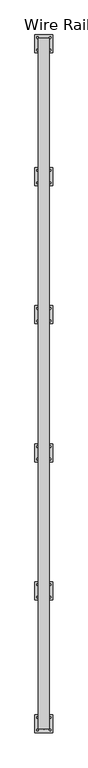
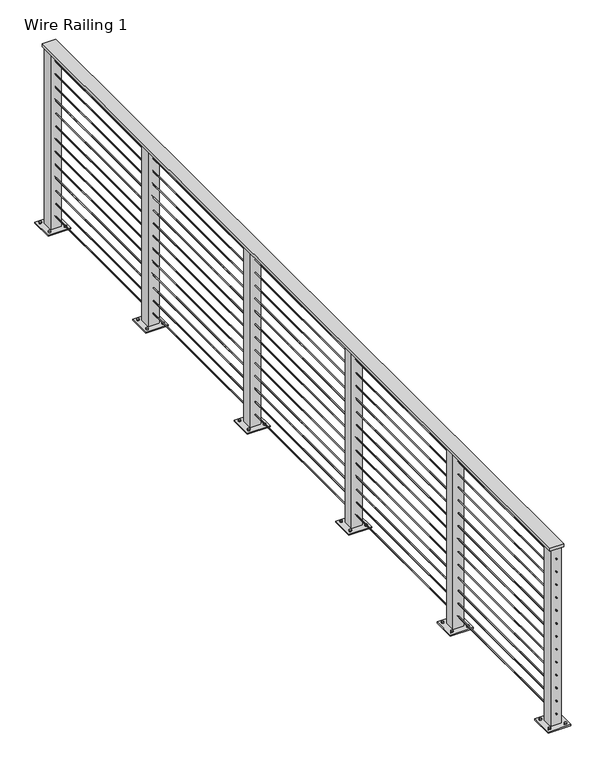
"""IFC4 building model written with IfcOpenShell, lengths in millimetres: railing geometry, Wire Railing 1."""

from ifc_helpers import new_model, si_unit, point, frame, frame_2d, origin, place, context, project, spatial, polyline, circle_curve, trimmed, segment, composite_curve, outline, extrude, source, transform, mapped, element, save


def wire_railing_1_036b5bdb(model_context):
    return source(origin(), model_context, "Body", "SweptSolid", [
        extrude(outline(polyline([(33186.6840778, 35113.0784511), (33262.8840778, 35113.0784511), (33262.8840778, 30205.3668167), (33186.6840778, 30205.3668167), (33186.6840778, 35113.0784511)])), frame((0.0, 0.0, 267442.95), z_axis=(0.0, 0.0, 1.0), x_axis=(1.0, 0.0, 0.0)), (0.0, 0.0, 1.0), 19.05),
        extrude(outline(composite_curve([segment(trimmed(circle_curve(frame_2d((267383.41875, 33224.7840778)), 2.38125), [point((267383.41875, 33227.1653278))], [point((267383.41875, 33222.4028278))], False, "CARTESIAN"), True, "CONTINUOUS"), segment(trimmed(circle_curve(frame_2d((267383.41875, 33224.7840778)), 2.38125), [point((267383.41875, 33222.4028278))], [point((267383.41875, 33227.1653278))], False, "CARTESIAN"), True, "CONTINUOUS")], self_intersect=False)), frame((0.0, 30205.3668167, 0.0), z_axis=(0.0, 1.0, 0.0), x_axis=(0.0, 0.0, 1.0)), (0.0, 0.0, 1.0), 4907.7116344),
        extrude(outline(composite_curve([segment(trimmed(circle_curve(frame_2d((267307.21875, 33224.7840778)), 2.38125), [point((267307.21875, 33227.1653278))], [point((267307.21875, 33222.4028278))], False, "CARTESIAN"), True, "CONTINUOUS"), segment(trimmed(circle_curve(frame_2d((267307.21875, 33224.7840778)), 2.38125), [point((267307.21875, 33222.4028278))], [point((267307.21875, 33227.1653278))], False, "CARTESIAN"), True, "CONTINUOUS")], self_intersect=False)), frame((0.0, 30205.3668167, 0.0), z_axis=(0.0, 1.0, 0.0), x_axis=(0.0, 0.0, 1.0)), (0.0, 0.0, 1.0), 4907.7116344),
        extrude(outline(composite_curve([segment(trimmed(circle_curve(frame_2d((267231.01875, 33224.7840778)), 2.38125), [point((267231.01875, 33227.1653278))], [point((267231.01875, 33222.4028278))], False, "CARTESIAN"), True, "CONTINUOUS"), segment(trimmed(circle_curve(frame_2d((267231.01875, 33224.7840778)), 2.38125), [point((267231.01875, 33222.4028278))], [point((267231.01875, 33227.1653278))], False, "CARTESIAN"), True, "CONTINUOUS")], self_intersect=False)), frame((0.0, 30205.3668167, 0.0), z_axis=(0.0, 1.0, 0.0), x_axis=(0.0, 0.0, 1.0)), (0.0, 0.0, 1.0), 4907.7116344),
        extrude(outline(composite_curve([segment(trimmed(circle_curve(frame_2d((267154.81875, 33224.7840778)), 2.38125), [point((267154.81875, 33227.1653278))], [point((267154.81875, 33222.4028278))], False, "CARTESIAN"), True, "CONTINUOUS"), segment(trimmed(circle_curve(frame_2d((267154.81875, 33224.7840778)), 2.38125), [point((267154.81875, 33222.4028278))], [point((267154.81875, 33227.1653278))], False, "CARTESIAN"), True, "CONTINUOUS")], self_intersect=False)), frame((0.0, 30205.3668167, 0.0), z_axis=(0.0, 1.0, 0.0), x_axis=(0.0, 0.0, 1.0)), (0.0, 0.0, 1.0), 4907.7116344),
        extrude(outline(composite_curve([segment(trimmed(circle_curve(frame_2d((267078.61875, 33224.7840778)), 2.38125), [point((267078.61875, 33227.1653278))], [point((267078.61875, 33222.4028278))], False, "CARTESIAN"), True, "CONTINUOUS"), segment(trimmed(circle_curve(frame_2d((267078.61875, 33224.7840778)), 2.38125), [point((267078.61875, 33222.4028278))], [point((267078.61875, 33227.1653278))], False, "CARTESIAN"), True, "CONTINUOUS")], self_intersect=False)), frame((0.0, 30205.3668167, 0.0), z_axis=(0.0, 1.0, 0.0), x_axis=(0.0, 0.0, 1.0)), (0.0, 0.0, 1.0), 4907.7116344),
        extrude(outline(composite_curve([segment(trimmed(circle_curve(frame_2d((267002.41875, 33224.7840778)), 2.38125), [point((267002.41875, 33227.1653278))], [point((267002.41875, 33222.4028278))], False, "CARTESIAN"), True, "CONTINUOUS"), segment(trimmed(circle_curve(frame_2d((267002.41875, 33224.7840778)), 2.38125), [point((267002.41875, 33222.4028278))], [point((267002.41875, 33227.1653278))], False, "CARTESIAN"), True, "CONTINUOUS")], self_intersect=False)), frame((0.0, 30205.3668167, 0.0), z_axis=(0.0, 1.0, 0.0), x_axis=(0.0, 0.0, 1.0)), (0.0, 0.0, 1.0), 4907.7116344),
        extrude(outline(composite_curve([segment(trimmed(circle_curve(frame_2d((266926.21875, 33224.7840778)), 2.38125), [point((266926.21875, 33227.1653278))], [point((266926.21875, 33222.4028278))], False, "CARTESIAN"), True, "CONTINUOUS"), segment(trimmed(circle_curve(frame_2d((266926.21875, 33224.7840778)), 2.38125), [point((266926.21875, 33222.4028278))], [point((266926.21875, 33227.1653278))], False, "CARTESIAN"), True, "CONTINUOUS")], self_intersect=False)), frame((0.0, 30205.3668167, 0.0), z_axis=(0.0, 1.0, 0.0), x_axis=(0.0, 0.0, 1.0)), (0.0, 0.0, 1.0), 4907.7116344),
        extrude(outline(composite_curve([segment(trimmed(circle_curve(frame_2d((266850.01875, 33224.7840778)), 2.38125), [point((266850.01875, 33227.1653278))], [point((266850.01875, 33222.4028278))], False, "CARTESIAN"), True, "CONTINUOUS"), segment(trimmed(circle_curve(frame_2d((266850.01875, 33224.7840778)), 2.38125), [point((266850.01875, 33222.4028278))], [point((266850.01875, 33227.1653278))], False, "CARTESIAN"), True, "CONTINUOUS")], self_intersect=False)), frame((0.0, 30205.3668167, 0.0), z_axis=(0.0, 1.0, 0.0), x_axis=(0.0, 0.0, 1.0)), (0.0, 0.0, 1.0), 4907.7116344),
        extrude(outline(composite_curve([segment(trimmed(circle_curve(frame_2d((266773.81875, 33224.7840778)), 2.38125), [point((266773.81875, 33227.1653278))], [point((266773.81875, 33222.4028278))], False, "CARTESIAN"), True, "CONTINUOUS"), segment(trimmed(circle_curve(frame_2d((266773.81875, 33224.7840778)), 2.38125), [point((266773.81875, 33222.4028278))], [point((266773.81875, 33227.1653278))], False, "CARTESIAN"), True, "CONTINUOUS")], self_intersect=False)), frame((0.0, 30205.3668167, 0.0), z_axis=(0.0, 1.0, 0.0), x_axis=(0.0, 0.0, 1.0)), (0.0, 0.0, 1.0), 4907.7116344),
        extrude(outline(composite_curve([segment(trimmed(circle_curve(frame_2d((266697.61875, 33224.7840778)), 2.38125), [point((266697.61875, 33227.1653278))], [point((266697.61875, 33222.4028278))], False, "CARTESIAN"), True, "CONTINUOUS"), segment(trimmed(circle_curve(frame_2d((266697.61875, 33224.7840778)), 2.38125), [point((266697.61875, 33222.4028278))], [point((266697.61875, 33227.1653278))], False, "CARTESIAN"), True, "CONTINUOUS")], self_intersect=False)), frame((0.0, 30205.3668167, 0.0), z_axis=(0.0, 1.0, 0.0), x_axis=(0.0, 0.0, 1.0)), (0.0, 0.0, 1.0), 4907.7116344),
        extrude(outline(composite_curve([segment(trimmed(circle_curve(frame_2d((266621.41875, 33224.7840778)), 2.38125), [point((266621.41875, 33227.1653278))], [point((266621.41875, 33222.4028278))], False, "CARTESIAN"), True, "CONTINUOUS"), segment(trimmed(circle_curve(frame_2d((266621.41875, 33224.7840778)), 2.38125), [point((266621.41875, 33222.4028278))], [point((266621.41875, 33227.1653278))], False, "CARTESIAN"), True, "CONTINUOUS")], self_intersect=False)), frame((0.0, 30205.3668167, 0.0), z_axis=(0.0, 1.0, 0.0), x_axis=(0.0, 0.0, 1.0)), (0.0, 0.0, 1.0), 4907.7116344),
        extrude(outline(composite_curve([segment(trimmed(circle_curve(frame_2d((266545.21875, 33224.7840778)), 2.38125), [point((266545.21875, 33227.1653278))], [point((266545.21875, 33222.4028278))], False, "CARTESIAN"), True, "CONTINUOUS"), segment(trimmed(circle_curve(frame_2d((266545.21875, 33224.7840778)), 2.38125), [point((266545.21875, 33222.4028278))], [point((266545.21875, 33227.1653278))], False, "CARTESIAN"), True, "CONTINUOUS")], self_intersect=False)), frame((0.0, 30205.3668167, 0.0), z_axis=(0.0, 1.0, 0.0), x_axis=(0.0, 0.0, 1.0)), (0.0, 0.0, 1.0), 4907.7116344),
        extrude(outline(composite_curve([segment(trimmed(circle_curve(frame_2d((266469.01875, 33224.7840778)), 2.38125), [point((266469.01875, 33227.1653278))], [point((266469.01875, 33222.4028278))], False, "CARTESIAN"), True, "CONTINUOUS"), segment(trimmed(circle_curve(frame_2d((266469.01875, 33224.7840778)), 2.38125), [point((266469.01875, 33222.4028278))], [point((266469.01875, 33227.1653278))], False, "CARTESIAN"), True, "CONTINUOUS")], self_intersect=False)), frame((0.0, 30205.3668167, 0.0), z_axis=(0.0, 1.0, 0.0), x_axis=(0.0, 0.0, 1.0)), (0.0, 0.0, 1.0), 4907.7116344),
        extrude(outline(composite_curve([segment(trimmed(circle_curve(frame_2d((33180.3340778, 31231.3591436)), 6.35), [point((33173.9840778, 31231.3591436))], [point((33186.6840778, 31231.3591436))], False, "CARTESIAN"), True, "CONTINUOUS"), segment(trimmed(circle_curve(frame_2d((33180.3340778, 31231.3591436)), 6.35), [point((33186.6840778, 31231.3591436))], [point((33173.9840778, 31231.3591436))], False, "CARTESIAN"), True, "CONTINUOUS")], self_intersect=False)), frame((0.0, 0.0, 266395.2), z_axis=(0.0, 0.0, 1.0), x_axis=(1.0, 0.0, 0.0)), (0.0, 0.0, 1.0), 12.7),
        extrude(outline(composite_curve([segment(trimmed(circle_curve(frame_2d((33269.2340778, 31231.3591436)), 6.35), [point((33262.8840778, 31231.3591436))], [point((33275.5840778, 31231.3591436))], False, "CARTESIAN"), True, "CONTINUOUS"), segment(trimmed(circle_curve(frame_2d((33269.2340778, 31231.3591436)), 6.35), [point((33275.5840778, 31231.3591436))], [point((33262.8840778, 31231.3591436))], False, "CARTESIAN"), True, "CONTINUOUS")], self_intersect=False)), frame((0.0, 0.0, 266395.2), z_axis=(0.0, 0.0, 1.0), x_axis=(1.0, 0.0, 0.0)), (0.0, 0.0, 1.0), 12.7),
        extrude(outline(composite_curve([segment(trimmed(circle_curve(frame_2d((33180.3340778, 31142.4591436)), 6.35), [point((33173.9840778, 31142.4591436))], [point((33186.6840778, 31142.4591436))], False, "CARTESIAN"), True, "CONTINUOUS"), segment(trimmed(circle_curve(frame_2d((33180.3340778, 31142.4591436)), 6.35), [point((33186.6840778, 31142.4591436))], [point((33173.9840778, 31142.4591436))], False, "CARTESIAN"), True, "CONTINUOUS")], self_intersect=False)), frame((0.0, 0.0, 266395.2), z_axis=(0.0, 0.0, 1.0), x_axis=(1.0, 0.0, 0.0)), (0.0, 0.0, 1.0), 12.7),
        extrude(outline(composite_curve([segment(trimmed(circle_curve(frame_2d((33269.2340778, 31142.4591436)), 6.35), [point((33262.8840778, 31142.4591436))], [point((33275.5840778, 31142.4591436))], False, "CARTESIAN"), True, "CONTINUOUS"), segment(trimmed(circle_curve(frame_2d((33269.2340778, 31142.4591436)), 6.35), [point((33275.5840778, 31142.4591436))], [point((33262.8840778, 31142.4591436))], False, "CARTESIAN"), True, "CONTINUOUS")], self_intersect=False)), frame((0.0, 0.0, 266395.2), z_axis=(0.0, 0.0, 1.0), x_axis=(1.0, 0.0, 0.0)), (0.0, 0.0, 1.0), 12.7),
        extrude(outline(polyline([(33288.2840778, 31250.4091436), (33288.2840778, 31123.4091436), (33161.2840778, 31123.4091436), (33161.2840778, 31250.4091436), (33288.2840778, 31250.4091436)])), frame((0.0, 0.0, 266395.2), z_axis=(0.0, 0.0, 1.0), x_axis=(1.0, 0.0, 0.0)), (0.0, 0.0, 1.0), 6.35),
        extrude(outline(polyline([(33254.9465778, 31217.0716436), (33254.9465778, 31156.7466436), (33194.6215778, 31156.7466436), (33194.6215778, 31217.0716436), (33254.9465778, 31217.0716436)]), holes=[polyline([(33248.5965778, 31210.7216436), (33200.9715778, 31210.7216436), (33200.9715778, 31163.0966436), (33248.5965778, 31163.0966436), (33248.5965778, 31210.7216436)])]), frame((0.0, 0.0, 266395.2), z_axis=(0.0, 0.0, 1.0), x_axis=(1.0, 0.0, 0.0)), (0.0, 0.0, 1.0), 1047.75),
        extrude(outline(composite_curve([segment(trimmed(circle_curve(frame_2d((33180.3340778, 32212.9014705)), 6.35), [point((33173.9840778, 32212.9014705))], [point((33186.6840778, 32212.9014705))], False, "CARTESIAN"), True, "CONTINUOUS"), segment(trimmed(circle_curve(frame_2d((33180.3340778, 32212.9014705)), 6.35), [point((33186.6840778, 32212.9014705))], [point((33173.9840778, 32212.9014705))], False, "CARTESIAN"), True, "CONTINUOUS")], self_intersect=False)), frame((0.0, 0.0, 266395.2), z_axis=(0.0, 0.0, 1.0), x_axis=(1.0, 0.0, 0.0)), (0.0, 0.0, 1.0), 12.7),
        extrude(outline(composite_curve([segment(trimmed(circle_curve(frame_2d((33269.2340778, 32212.9014705)), 6.35), [point((33262.8840778, 32212.9014705))], [point((33275.5840778, 32212.9014705))], False, "CARTESIAN"), True, "CONTINUOUS"), segment(trimmed(circle_curve(frame_2d((33269.2340778, 32212.9014705)), 6.35), [point((33275.5840778, 32212.9014705))], [point((33262.8840778, 32212.9014705))], False, "CARTESIAN"), True, "CONTINUOUS")], self_intersect=False)), frame((0.0, 0.0, 266395.2), z_axis=(0.0, 0.0, 1.0), x_axis=(1.0, 0.0, 0.0)), (0.0, 0.0, 1.0), 12.7),
        extrude(outline(composite_curve([segment(trimmed(circle_curve(frame_2d((33180.3340778, 32124.0014705)), 6.35), [point((33173.9840778, 32124.0014705))], [point((33186.6840778, 32124.0014705))], False, "CARTESIAN"), True, "CONTINUOUS"), segment(trimmed(circle_curve(frame_2d((33180.3340778, 32124.0014705)), 6.35), [point((33186.6840778, 32124.0014705))], [point((33173.9840778, 32124.0014705))], False, "CARTESIAN"), True, "CONTINUOUS")], self_intersect=False)), frame((0.0, 0.0, 266395.2), z_axis=(0.0, 0.0, 1.0), x_axis=(1.0, 0.0, 0.0)), (0.0, 0.0, 1.0), 12.7),
        extrude(outline(composite_curve([segment(trimmed(circle_curve(frame_2d((33269.2340778, 32124.0014705)), 6.35), [point((33262.8840778, 32124.0014705))], [point((33275.5840778, 32124.0014705))], False, "CARTESIAN"), True, "CONTINUOUS"), segment(trimmed(circle_curve(frame_2d((33269.2340778, 32124.0014705)), 6.35), [point((33275.5840778, 32124.0014705))], [point((33262.8840778, 32124.0014705))], False, "CARTESIAN"), True, "CONTINUOUS")], self_intersect=False)), frame((0.0, 0.0, 266395.2), z_axis=(0.0, 0.0, 1.0), x_axis=(1.0, 0.0, 0.0)), (0.0, 0.0, 1.0), 12.7),
        extrude(outline(polyline([(33288.2840778, 32231.9514705), (33288.2840778, 32104.9514705), (33161.2840778, 32104.9514705), (33161.2840778, 32231.9514705), (33288.2840778, 32231.9514705)])), frame((0.0, 0.0, 266395.2), z_axis=(0.0, 0.0, 1.0), x_axis=(1.0, 0.0, 0.0)), (0.0, 0.0, 1.0), 6.35),
        extrude(outline(polyline([(33254.9465778, 32198.6139705), (33254.9465778, 32138.2889705), (33194.6215778, 32138.2889705), (33194.6215778, 32198.6139705), (33254.9465778, 32198.6139705)]), holes=[polyline([(33248.5965778, 32192.2639705), (33200.9715778, 32192.2639705), (33200.9715778, 32144.6389705), (33248.5965778, 32144.6389705), (33248.5965778, 32192.2639705)])]), frame((0.0, 0.0, 266395.2), z_axis=(0.0, 0.0, 1.0), x_axis=(1.0, 0.0, 0.0)), (0.0, 0.0, 1.0), 1047.75),
        extrude(outline(composite_curve([segment(trimmed(circle_curve(frame_2d((33180.3340778, 33194.4437973)), 6.35), [point((33173.9840778, 33194.4437973))], [point((33186.6840778, 33194.4437973))], False, "CARTESIAN"), True, "CONTINUOUS"), segment(trimmed(circle_curve(frame_2d((33180.3340778, 33194.4437973)), 6.35), [point((33186.6840778, 33194.4437973))], [point((33173.9840778, 33194.4437973))], False, "CARTESIAN"), True, "CONTINUOUS")], self_intersect=False)), frame((0.0, 0.0, 266395.2), z_axis=(0.0, 0.0, 1.0), x_axis=(1.0, 0.0, 0.0)), (0.0, 0.0, 1.0), 12.7),
        extrude(outline(composite_curve([segment(trimmed(circle_curve(frame_2d((33269.2340778, 33194.4437973)), 6.35), [point((33262.8840778, 33194.4437973))], [point((33275.5840778, 33194.4437973))], False, "CARTESIAN"), True, "CONTINUOUS"), segment(trimmed(circle_curve(frame_2d((33269.2340778, 33194.4437973)), 6.35), [point((33275.5840778, 33194.4437973))], [point((33262.8840778, 33194.4437973))], False, "CARTESIAN"), True, "CONTINUOUS")], self_intersect=False)), frame((0.0, 0.0, 266395.2), z_axis=(0.0, 0.0, 1.0), x_axis=(1.0, 0.0, 0.0)), (0.0, 0.0, 1.0), 12.7),
        extrude(outline(composite_curve([segment(trimmed(circle_curve(frame_2d((33180.3340778, 33105.5437973)), 6.35), [point((33173.9840778, 33105.5437973))], [point((33186.6840778, 33105.5437973))], False, "CARTESIAN"), True, "CONTINUOUS"), segment(trimmed(circle_curve(frame_2d((33180.3340778, 33105.5437973)), 6.35), [point((33186.6840778, 33105.5437973))], [point((33173.9840778, 33105.5437973))], False, "CARTESIAN"), True, "CONTINUOUS")], self_intersect=False)), frame((0.0, 0.0, 266395.2), z_axis=(0.0, 0.0, 1.0), x_axis=(1.0, 0.0, 0.0)), (0.0, 0.0, 1.0), 12.7),
        extrude(outline(composite_curve([segment(trimmed(circle_curve(frame_2d((33269.2340778, 33105.5437973)), 6.35), [point((33262.8840778, 33105.5437973))], [point((33275.5840778, 33105.5437973))], False, "CARTESIAN"), True, "CONTINUOUS"), segment(trimmed(circle_curve(frame_2d((33269.2340778, 33105.5437973)), 6.35), [point((33275.5840778, 33105.5437973))], [point((33262.8840778, 33105.5437973))], False, "CARTESIAN"), True, "CONTINUOUS")], self_intersect=False)), frame((0.0, 0.0, 266395.2), z_axis=(0.0, 0.0, 1.0), x_axis=(1.0, 0.0, 0.0)), (0.0, 0.0, 1.0), 12.7),
        extrude(outline(polyline([(33288.2840778, 33213.4937973), (33288.2840778, 33086.4937973), (33161.2840778, 33086.4937973), (33161.2840778, 33213.4937973), (33288.2840778, 33213.4937973)])), frame((0.0, 0.0, 266395.2), z_axis=(0.0, 0.0, 1.0), x_axis=(1.0, 0.0, 0.0)), (0.0, 0.0, 1.0), 6.35),
        extrude(outline(polyline([(33254.9465778, 33180.1562973), (33254.9465778, 33119.8312973), (33194.6215778, 33119.8312973), (33194.6215778, 33180.1562973), (33254.9465778, 33180.1562973)]), holes=[polyline([(33248.5965778, 33173.8062973), (33200.9715778, 33173.8062973), (33200.9715778, 33126.1812973), (33248.5965778, 33126.1812973), (33248.5965778, 33173.8062973)])]), frame((0.0, 0.0, 266395.2), z_axis=(0.0, 0.0, 1.0), x_axis=(1.0, 0.0, 0.0)), (0.0, 0.0, 1.0), 1047.75),
        extrude(outline(composite_curve([segment(trimmed(circle_curve(frame_2d((33180.3340778, 34175.9861242)), 6.35), [point((33173.9840778, 34175.9861242))], [point((33186.6840778, 34175.9861242))], False, "CARTESIAN"), True, "CONTINUOUS"), segment(trimmed(circle_curve(frame_2d((33180.3340778, 34175.9861242)), 6.35), [point((33186.6840778, 34175.9861242))], [point((33173.9840778, 34175.9861242))], False, "CARTESIAN"), True, "CONTINUOUS")], self_intersect=False)), frame((0.0, 0.0, 266395.2), z_axis=(0.0, 0.0, 1.0), x_axis=(1.0, 0.0, 0.0)), (0.0, 0.0, 1.0), 12.7),
        extrude(outline(composite_curve([segment(trimmed(circle_curve(frame_2d((33269.2340778, 34175.9861242)), 6.35), [point((33262.8840778, 34175.9861242))], [point((33275.5840778, 34175.9861242))], False, "CARTESIAN"), True, "CONTINUOUS"), segment(trimmed(circle_curve(frame_2d((33269.2340778, 34175.9861242)), 6.35), [point((33275.5840778, 34175.9861242))], [point((33262.8840778, 34175.9861242))], False, "CARTESIAN"), True, "CONTINUOUS")], self_intersect=False)), frame((0.0, 0.0, 266395.2), z_axis=(0.0, 0.0, 1.0), x_axis=(1.0, 0.0, 0.0)), (0.0, 0.0, 1.0), 12.7),
        extrude(outline(composite_curve([segment(trimmed(circle_curve(frame_2d((33180.3340778, 34087.0861242)), 6.35), [point((33173.9840778, 34087.0861242))], [point((33186.6840778, 34087.0861242))], False, "CARTESIAN"), True, "CONTINUOUS"), segment(trimmed(circle_curve(frame_2d((33180.3340778, 34087.0861242)), 6.35), [point((33186.6840778, 34087.0861242))], [point((33173.9840778, 34087.0861242))], False, "CARTESIAN"), True, "CONTINUOUS")], self_intersect=False)), frame((0.0, 0.0, 266395.2), z_axis=(0.0, 0.0, 1.0), x_axis=(1.0, 0.0, 0.0)), (0.0, 0.0, 1.0), 12.7),
        extrude(outline(composite_curve([segment(trimmed(circle_curve(frame_2d((33269.2340778, 34087.0861242)), 6.35), [point((33262.8840778, 34087.0861242))], [point((33275.5840778, 34087.0861242))], False, "CARTESIAN"), True, "CONTINUOUS"), segment(trimmed(circle_curve(frame_2d((33269.2340778, 34087.0861242)), 6.35), [point((33275.5840778, 34087.0861242))], [point((33262.8840778, 34087.0861242))], False, "CARTESIAN"), True, "CONTINUOUS")], self_intersect=False)), frame((0.0, 0.0, 266395.2), z_axis=(0.0, 0.0, 1.0), x_axis=(1.0, 0.0, 0.0)), (0.0, 0.0, 1.0), 12.7),
        extrude(outline(polyline([(33288.2840778, 34195.0361242), (33288.2840778, 34068.0361242), (33161.2840778, 34068.0361242), (33161.2840778, 34195.0361242), (33288.2840778, 34195.0361242)])), frame((0.0, 0.0, 266395.2), z_axis=(0.0, 0.0, 1.0), x_axis=(1.0, 0.0, 0.0)), (0.0, 0.0, 1.0), 6.35),
        extrude(outline(polyline([(33254.9465778, 34161.6986242), (33254.9465778, 34101.3736242), (33194.6215778, 34101.3736242), (33194.6215778, 34161.6986242), (33254.9465778, 34161.6986242)]), holes=[polyline([(33248.5965778, 34155.3486242), (33200.9715778, 34155.3486242), (33200.9715778, 34107.7236242), (33248.5965778, 34107.7236242), (33248.5965778, 34155.3486242)])]), frame((0.0, 0.0, 266395.2), z_axis=(0.0, 0.0, 1.0), x_axis=(1.0, 0.0, 0.0)), (0.0, 0.0, 1.0), 1047.75),
        extrude(outline(composite_curve([segment(trimmed(circle_curve(frame_2d((33180.3340778, 30287.9168167)), 6.35), [point((33173.9840778, 30287.9168167))], [point((33186.6840778, 30287.9168167))], False, "CARTESIAN"), True, "CONTINUOUS"), segment(trimmed(circle_curve(frame_2d((33180.3340778, 30287.9168167)), 6.35), [point((33186.6840778, 30287.9168167))], [point((33173.9840778, 30287.9168167))], False, "CARTESIAN"), True, "CONTINUOUS")], self_intersect=False)), frame((0.0, 0.0, 266395.2), z_axis=(0.0, 0.0, 1.0), x_axis=(1.0, 0.0, 0.0)), (0.0, 0.0, 1.0), 12.7),
        extrude(outline(composite_curve([segment(trimmed(circle_curve(frame_2d((33269.2340778, 30287.9168167)), 6.35), [point((33262.8840778, 30287.9168167))], [point((33275.5840778, 30287.9168167))], False, "CARTESIAN"), True, "CONTINUOUS"), segment(trimmed(circle_curve(frame_2d((33269.2340778, 30287.9168167)), 6.35), [point((33275.5840778, 30287.9168167))], [point((33262.8840778, 30287.9168167))], False, "CARTESIAN"), True, "CONTINUOUS")], self_intersect=False)), frame((0.0, 0.0, 266395.2), z_axis=(0.0, 0.0, 1.0), x_axis=(1.0, 0.0, 0.0)), (0.0, 0.0, 1.0), 12.7),
        extrude(outline(composite_curve([segment(trimmed(circle_curve(frame_2d((33180.3340778, 30199.0168167)), 6.35), [point((33173.9840778, 30199.0168167))], [point((33186.6840778, 30199.0168167))], False, "CARTESIAN"), True, "CONTINUOUS"), segment(trimmed(circle_curve(frame_2d((33180.3340778, 30199.0168167)), 6.35), [point((33186.6840778, 30199.0168167))], [point((33173.9840778, 30199.0168167))], False, "CARTESIAN"), True, "CONTINUOUS")], self_intersect=False)), frame((0.0, 0.0, 266395.2), z_axis=(0.0, 0.0, 1.0), x_axis=(1.0, 0.0, 0.0)), (0.0, 0.0, 1.0), 12.7),
        extrude(outline(composite_curve([segment(trimmed(circle_curve(frame_2d((33269.2340778, 30199.0168167)), 6.35), [point((33262.8840778, 30199.0168167))], [point((33275.5840778, 30199.0168167))], False, "CARTESIAN"), True, "CONTINUOUS"), segment(trimmed(circle_curve(frame_2d((33269.2340778, 30199.0168167)), 6.35), [point((33275.5840778, 30199.0168167))], [point((33262.8840778, 30199.0168167))], False, "CARTESIAN"), True, "CONTINUOUS")], self_intersect=False)), frame((0.0, 0.0, 266395.2), z_axis=(0.0, 0.0, 1.0), x_axis=(1.0, 0.0, 0.0)), (0.0, 0.0, 1.0), 12.7),
        extrude(outline(polyline([(33288.2840778, 30306.9668167), (33288.2840778, 30179.9668167), (33161.2840778, 30179.9668167), (33161.2840778, 30306.9668167), (33288.2840778, 30306.9668167)])), frame((0.0, 0.0, 266395.2), z_axis=(0.0, 0.0, 1.0), x_axis=(1.0, 0.0, 0.0)), (0.0, 0.0, 1.0), 6.35),
        extrude(outline(polyline([(33254.9465778, 30273.6293167), (33254.9465778, 30213.3043167), (33194.6215778, 30213.3043167), (33194.6215778, 30273.6293167), (33254.9465778, 30273.6293167)]), holes=[polyline([(33248.5965778, 30267.2793167), (33200.9715778, 30267.2793167), (33200.9715778, 30219.6543167), (33248.5965778, 30219.6543167), (33248.5965778, 30267.2793167)])]), frame((0.0, 0.0, 266395.2), z_axis=(0.0, 0.0, 1.0), x_axis=(1.0, 0.0, 0.0)), (0.0, 0.0, 1.0), 1047.75),
        extrude(outline(composite_curve([segment(trimmed(circle_curve(frame_2d((33180.3340778, 35119.4284511)), 6.35), [point((33173.9840778, 35119.4284511))], [point((33186.6840778, 35119.4284511))], False, "CARTESIAN"), True, "CONTINUOUS"), segment(trimmed(circle_curve(frame_2d((33180.3340778, 35119.4284511)), 6.35), [point((33186.6840778, 35119.4284511))], [point((33173.9840778, 35119.4284511))], False, "CARTESIAN"), True, "CONTINUOUS")], self_intersect=False)), frame((0.0, 0.0, 266395.2), z_axis=(0.0, 0.0, 1.0), x_axis=(1.0, 0.0, 0.0)), (0.0, 0.0, 1.0), 12.7),
        extrude(outline(composite_curve([segment(trimmed(circle_curve(frame_2d((33269.2340778, 35119.4284511)), 6.35), [point((33262.8840778, 35119.4284511))], [point((33275.5840778, 35119.4284511))], False, "CARTESIAN"), True, "CONTINUOUS"), segment(trimmed(circle_curve(frame_2d((33269.2340778, 35119.4284511)), 6.35), [point((33275.5840778, 35119.4284511))], [point((33262.8840778, 35119.4284511))], False, "CARTESIAN"), True, "CONTINUOUS")], self_intersect=False)), frame((0.0, 0.0, 266395.2), z_axis=(0.0, 0.0, 1.0), x_axis=(1.0, 0.0, 0.0)), (0.0, 0.0, 1.0), 12.7),
        extrude(outline(composite_curve([segment(trimmed(circle_curve(frame_2d((33180.3340778, 35030.5284511)), 6.35), [point((33173.9840778, 35030.5284511))], [point((33186.6840778, 35030.5284511))], False, "CARTESIAN"), True, "CONTINUOUS"), segment(trimmed(circle_curve(frame_2d((33180.3340778, 35030.5284511)), 6.35), [point((33186.6840778, 35030.5284511))], [point((33173.9840778, 35030.5284511))], False, "CARTESIAN"), True, "CONTINUOUS")], self_intersect=False)), frame((0.0, 0.0, 266395.2), z_axis=(0.0, 0.0, 1.0), x_axis=(1.0, 0.0, 0.0)), (0.0, 0.0, 1.0), 12.7),
        extrude(outline(composite_curve([segment(trimmed(circle_curve(frame_2d((33269.2340778, 35030.5284511)), 6.35), [point((33262.8840778, 35030.5284511))], [point((33275.5840778, 35030.5284511))], False, "CARTESIAN"), True, "CONTINUOUS"), segment(trimmed(circle_curve(frame_2d((33269.2340778, 35030.5284511)), 6.35), [point((33275.5840778, 35030.5284511))], [point((33262.8840778, 35030.5284511))], False, "CARTESIAN"), True, "CONTINUOUS")], self_intersect=False)), frame((0.0, 0.0, 266395.2), z_axis=(0.0, 0.0, 1.0), x_axis=(1.0, 0.0, 0.0)), (0.0, 0.0, 1.0), 12.7),
        extrude(outline(polyline([(33288.2840778, 35138.4784511), (33288.2840778, 35011.4784511), (33161.2840778, 35011.4784511), (33161.2840778, 35138.4784511), (33288.2840778, 35138.4784511)])), frame((0.0, 0.0, 266395.2), z_axis=(0.0, 0.0, 1.0), x_axis=(1.0, 0.0, 0.0)), (0.0, 0.0, 1.0), 6.35),
        extrude(outline(polyline([(33254.9465778, 35105.1409511), (33254.9465778, 35044.8159511), (33194.6215778, 35044.8159511), (33194.6215778, 35105.1409511), (33254.9465778, 35105.1409511)]), holes=[polyline([(33248.5965778, 35098.7909511), (33200.9715778, 35098.7909511), (33200.9715778, 35051.1659511), (33248.5965778, 35051.1659511), (33248.5965778, 35098.7909511)])]), frame((0.0, 0.0, 266395.2), z_axis=(0.0, 0.0, 1.0), x_axis=(1.0, 0.0, 0.0)), (0.0, 0.0, 1.0), 1047.75),
    ])


if __name__ == "__main__":
    model = new_model("IFC4")
    model_context = context("Model", 3, world=origin())
    ifc_project = project(units=[si_unit("LENGTHUNIT", "METRE", prefix="MILLI")], contexts=[model_context])
    site = spatial("IfcSite", under=ifc_project)
    building = spatial("IfcBuilding", under=site)
    placement = place(None, origin())
    wire_railing_1_shape = wire_railing_1_036b5bdb(model_context)
    element("IfcRailing", 1, ObjectType="Wire Railing 1", at=placement, inside=building, context=model_context, shape_type="MappedRepresentation", body=[
        mapped(wire_railing_1_shape, transform((0.0, 0.0, 0.0), x_axis=(1.0, 0.0, 0.0), y_axis=(0.0, 1.0, 0.0), z_axis=(0.0, 0.0, 1.0))),
    ])
    save(model, "model.ifc")

# Revit data of these elements
# Element 1 (IfcRailing, "Wire Railing 1")
#   Materials on its faces: "2 1/2\" X 2 1/2\" ALUM. SQUARE POST (38\" O.C. MAX)", "WIRE RAILING (3\" O.C.)", "ALUM. PLATE TOP RAIL"
# Materials
#   "2 1/2\" X 2 1/2\" ALUM. SQUARE POST (38\" O.C. MAX)": class "Metal", colour RGB 244 244 244, transparency 0, Manufacturer = "Kawneer", URL = "http://www.kawneer.com/kawneer/north_america/en/home.asp", Cost = 0
#   "WIRE RAILING (3\" O.C.)": class "Metal", colour RGB 244 244 244, transparency 0, Manufacturer = "Kawneer", URL = "http://www.kawneer.com/kawneer/north_america/en/home.asp", Cost = 0
#   "ALUM. PLATE TOP RAIL": class "Metal", colour RGB 244 244 244, transparency 0, Manufacturer = "Kawneer", URL = "http://www.kawneer.com/kawneer/north_america/en/home.asp", Cost = 0
